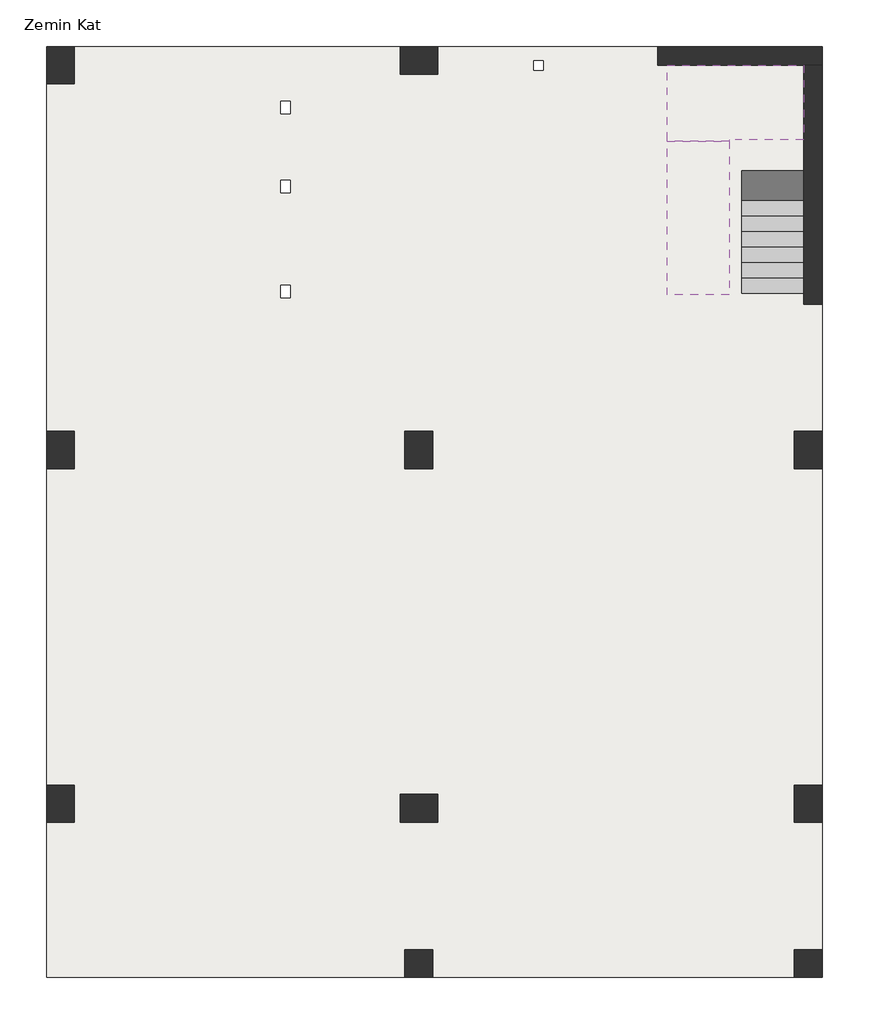
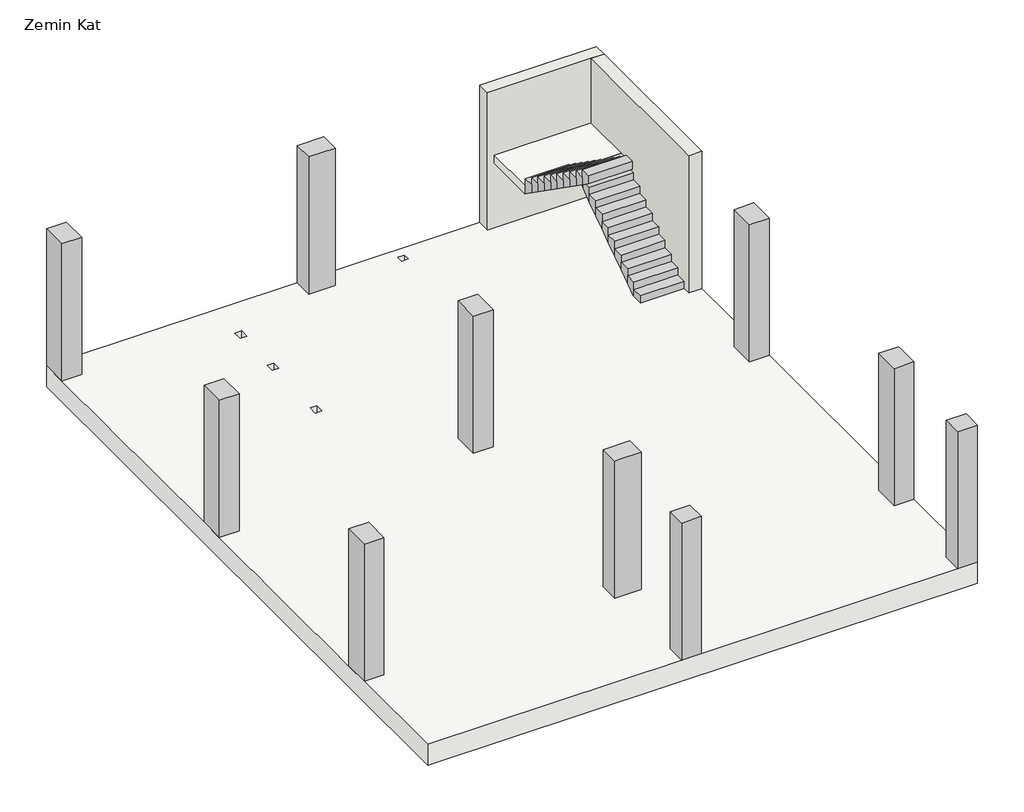
# One storey: 10 columns, 2 slabs, 2 stair flights, 2 walls.
"""IFC4 building model written with IfcOpenShell, lengths in millimetres."""

from ifc_helpers import new_model, si_unit, frame, origin, place, context, project, spatial, polyline, outline, extrude, faceted_brep, element, save

model = new_model("IFC4")

# Units and contexts
model_context = context("Model", 3, world=origin())
ifc_project = project(units=[si_unit("LENGTHUNIT", "METRE", prefix="MILLI")], contexts=[model_context])

# Site, building, storey
site = spatial("IfcSite", under=ifc_project)
building = spatial("IfcBuilding", under=site)
storey = spatial("IfcBuildingStorey", under=building, Name="Zemin Kat", Elevation=93780.0)

# Columns
placement = place(None, origin())
element("IfcColumn", 1, ObjectType="M_Concrete-Rectangular-Column : 450 x 450mm", at=placement, inside=storey, context=model_context, shape_type="SweptSolid", body=[
    extrude(outline(polyline([(-8954.0485128, -6221.7095574), (-9404.0485128, -6221.7095574), (-9404.0485128, -5771.7095574), (-8954.0485128, -5771.7095574), (-8954.0485128, -6221.7095574)])), frame((0.0, 0.0, 93780.0), z_axis=(0.0, 0.0, 1.0), x_axis=(1.0, 0.0, 0.0)), (0.0, 0.0, 1.0), 3300.0),
])
element("IfcColumn", 2, ObjectType="M_Concrete-Rectangular-Column : 450 x 450mm", at=placement, inside=storey, context=model_context, shape_type="SweptSolid", body=[
    extrude(outline(polyline([(-3129.0485128, -6221.7095574), (-3129.0485128, -5771.7095574), (-2679.0485128, -5771.7095574), (-2679.0485128, -6221.7095574), (-3129.0485128, -6221.7095574)])), frame((0.0, 0.0, 93780.0), z_axis=(0.0, 0.0, 1.0), x_axis=(1.0, 0.0, 0.0)), (0.0, 0.0, 1.0), 3300.0),
])
element("IfcColumn", 3, ObjectType="M_Concrete-Rectangular-Column : 450 x 600mm", at=placement, inside=storey, context=model_context, shape_type="SweptSolid", body=[
    extrude(outline(polyline([(-15179.0485128, -3721.7095574), (-15179.0485128, -3121.7095574), (-14729.0485128, -3121.7095574), (-14729.0485128, -3721.7095574), (-15179.0485128, -3721.7095574)])), frame((0.0, 0.0, 93780.0), z_axis=(0.0, 0.0, 1.0), x_axis=(1.0, 0.0, 0.0)), (0.0, 0.0, 1.0), 3300.0),
])
element("IfcColumn", 4, ObjectType="M_Concrete-Rectangular-Column : 450 x 600mm", at=placement, inside=storey, context=model_context, shape_type="SweptSolid", body=[
    extrude(outline(polyline([(-15179.0485128, 1978.2904426), (-15179.0485128, 2578.2904426), (-14729.0485128, 2578.2904426), (-14729.0485128, 1978.2904426), (-15179.0485128, 1978.2904426)])), frame((0.0, 0.0, 93780.0), z_axis=(0.0, 0.0, 1.0), x_axis=(1.0, 0.0, 0.0)), (0.0, 0.0, 1.0), 3300.0),
])
element("IfcColumn", 5, ObjectType="M_Concrete-Rectangular-Column : 450 x 600mm", at=placement, inside=storey, context=model_context, shape_type="SweptSolid", body=[
    extrude(outline(polyline([(-15179.0485128, 8178.2904426), (-15179.0485128, 8778.2904426), (-14729.0485128, 8778.2904426), (-14729.0485128, 8178.2904426), (-15179.0485128, 8178.2904426)])), frame((0.0, 0.0, 93780.0), z_axis=(0.0, 0.0, 1.0), x_axis=(1.0, 0.0, 0.0)), (0.0, 0.0, 1.0), 3300.0),
])
element("IfcColumn", 6, ObjectType="M_Concrete-Rectangular-Column : 450 x 600mm", at=placement, inside=storey, context=model_context, shape_type="Brep", body=[
    faceted_brep([(-8879.0485128, -3721.7095574, 93780.0), (-9479.0485128, -3721.7095574, 93780.0), (-9479.0485128, -3271.7095574, 93780.0), (-8879.0485128, -3271.7095574, 93780.0), (-8879.0485128, -3721.7095574, 97080.0), (-9404.0485128, -3721.7095574, 97080.0), (-9479.0485128, -3721.7095574, 97080.0), (-9479.0485128, -3271.7095574, 97080.0), (-8879.0485128, -3271.7095574, 97080.0)], [[[0, 1, 2, 3]], [[1, 0, 4, 5, 6]], [[2, 1, 6, 7]], [[3, 2, 7, 8]], [[0, 3, 8, 4]], [[6, 5, 4, 8, 7]]]),
])
element("IfcColumn", 7, ObjectType="M_Concrete-Rectangular-Column : 450 x 600mm", at=placement, inside=storey, context=model_context, shape_type="SweptSolid", body=[
    extrude(outline(polyline([(-9404.0485128, 1978.2904426), (-9404.0485128, 2578.2904426), (-8954.0485128, 2578.2904426), (-8954.0485128, 1978.2904426), (-9404.0485128, 1978.2904426)])), frame((0.0, 0.0, 93780.0), z_axis=(0.0, 0.0, 1.0), x_axis=(1.0, 0.0, 0.0)), (0.0, 0.0, 1.0), 3300.0),
])
element("IfcColumn", 8, ObjectType="M_Concrete-Rectangular-Column : 450 x 600mm", at=placement, inside=storey, context=model_context, shape_type="SweptSolid", body=[
    extrude(outline(polyline([(-8879.0485128, 8328.2904426), (-9479.0485128, 8328.2904426), (-9479.0485128, 8778.2904426), (-8879.0485128, 8778.2904426), (-8879.0485128, 8328.2904426)])), frame((0.0, 0.0, 93780.0), z_axis=(0.0, 0.0, 1.0), x_axis=(1.0, 0.0, 0.0)), (0.0, 0.0, 1.0), 3300.0),
])
element("IfcColumn", 9, ObjectType="M_Concrete-Rectangular-Column : 450 x 600mm", at=placement, inside=storey, context=model_context, shape_type="Brep", body=[
    faceted_brep([(-3129.0485128, -3721.7095574, 93780.0), (-3129.0485128, -3121.7095574, 93780.0), (-2679.0485128, -3121.7095574, 93780.0), (-2679.0485128, -3721.7095574, 93780.0), (-3129.0485128, -3721.7095574, 97080.0), (-3129.0485128, -3121.7095574, 97080.0), (-3129.0485128, -3121.7095574, 96680.0), (-2679.0485128, -3121.7095574, 97080.0), (-2679.0485128, -3121.7095574, 96680.0), (-2679.0485128, -3721.7095574, 97080.0)], [[[0, 1, 2, 3]], [[1, 0, 4, 5, 6]], [[2, 1, 6, 5, 7, 8]], [[3, 2, 8, 7, 9]], [[0, 3, 9, 4]], [[5, 4, 9, 7]]]),
])
element("IfcColumn", 10, ObjectType="M_Concrete-Rectangular-Column : 450 x 600mm", at=placement, inside=storey, context=model_context, shape_type="SweptSolid", body=[
    extrude(outline(polyline([(-3129.0485128, 1978.2904426), (-3129.0485128, 2578.2904426), (-2679.0485128, 2578.2904426), (-2679.0485128, 1978.2904426), (-3129.0485128, 1978.2904426)])), frame((0.0, 0.0, 93780.0), z_axis=(0.0, 0.0, 1.0), x_axis=(1.0, 0.0, 0.0)), (0.0, 0.0, 1.0), 3300.0),
])

# Slabs
element("IfcSlab", 11, ObjectType="200 mm Thickness", at=placement, inside=storey, context=model_context, shape_type="Brep", body=[
    faceted_brep([(-3979.0485128, 7278.2904426, 95530.0), (-2979.0485128, 7278.2904426, 95530.0), (-2979.0485128, 7279.1452058, 95530.0), (-2979.0485128, 8478.2904426, 95530.0), (-5179.0485128, 8478.2904426, 95530.0), (-5179.0485128, 7278.2904426, 95530.0), (-5179.0485128, 7277.4356794, 95530.0), (-5179.0485128, 7253.2904426, 95530.0), (-4179.0485128, 7253.2904426, 95530.0), (-4179.0485128, 7277.4356794, 95530.0), (-4179.0485128, 7278.2904426, 95530.0), (-5179.0485128, 8478.2904426, 95330.0), (-5179.0485128, 7278.2904426, 95330.0), (-5179.0485128, 7253.2904426, 95346.9016658), (-4179.0485128, 7253.2904426, 95346.9016658), (-5179.0485128, 7277.4356794, 95330.0), (-4179.0485128, 7278.2904426, 95330.0), (-3979.0485128, 7278.2904426, 95330.0), (-2979.0485128, 7278.2904426, 95329.4016658), (-2979.0485128, 7279.1452058, 95330.0), (-2979.0485128, 8478.2904426, 95330.0), (-3979.0485128, 7279.1452058, 95330.0), (-4179.0485128, 7277.4356794, 95330.0), (-3979.0485128, 7278.2904426, 95329.4016658)], [[[0, 1, 2, 3, 4, 5, 6, 7, 8, 9, 10]], [[5, 4, 11, 12]], [[8, 7, 13, 14]], [[5, 12, 15, 13, 7, 6]], [[0, 10, 16, 17]], [[1, 18, 19, 20, 3, 2]], [[19, 21, 17, 16, 22, 15, 12, 11, 20]], [[1, 0, 17, 23, 18]], [[4, 3, 20, 11]], [[8, 14, 22, 16, 10, 9]], [[21, 19, 18, 23]], [[17, 21, 23]], [[15, 22, 14, 13]]]),
])
element("IfcSlab", 12, ObjectType="Generic 500mm", at=placement, inside=storey, context=model_context, shape_type="Brep", body=[
    faceted_brep([(-2679.0485128, 8778.2904426, 93280.0), (-2679.0485128, -6221.7095574, 93280.0), (-15179.0485128, -6221.7095574, 93280.0), (-15179.0485128, 8778.2904426, 93280.0), (-11404.0485128, 6624.8694152, 93280.0), (-11404.0485128, 6424.8694152, 93280.0), (-11254.0485128, 6424.8694152, 93280.0), (-11254.0485128, 6624.8694152, 93280.0), (-11404.0485128, 4933.2654426, 93280.0), (-11404.0485128, 4733.2654426, 93280.0), (-11254.0485128, 4733.2654426, 93280.0), (-11254.0485128, 4933.2654426, 93280.0), (-11404.0485128, 7898.2904426, 93280.0), (-11404.0485128, 7698.2904426, 93280.0), (-11254.0485128, 7698.2904426, 93280.0), (-11254.0485128, 7898.2904426, 93280.0), (-7326.5485128, 8548.2904426, 93280.0), (-7326.5485128, 8398.2904426, 93280.0), (-7176.5485128, 8398.2904426, 93280.0), (-7176.5485128, 8548.2904426, 93280.0), (-2679.0485128, -6221.7095574, 93780.0), (-2679.0485128, -5771.7095574, 93780.0), (-2679.0485128, -3721.7095574, 93780.0), (-2679.0485128, -3121.7095574, 93780.0), (-2679.0485128, 1978.2904426, 93780.0), (-2679.0485128, 2578.2904426, 93780.0), (-2679.0485128, 8778.2904426, 93780.0), (-8879.0485128, 8778.2904426, 93780.0), (-9479.0485128, 8778.2904426, 93780.0), (-14729.0485128, 8778.2904426, 93780.0), (-15179.0485128, 8778.2904426, 93780.0), (-15179.0485128, 8178.2904426, 93780.0), (-15179.0485128, 2578.2904426, 93780.0), (-15179.0485128, 1978.2904426, 93780.0), (-15179.0485128, -3121.7095574, 93780.0), (-15179.0485128, -3721.7095574, 93780.0), (-15179.0485128, -6221.7095574, 93780.0), (-9404.0485128, -6221.7095574, 93780.0), (-8954.0485128, -6221.7095574, 93780.0), (-3129.0485128, -6221.7095574, 93780.0), (-11404.0485128, 6424.8694152, 93780.0), (-11404.0485128, 6624.8694152, 93780.0), (-11254.0485128, 6624.8694152, 93780.0), (-11254.0485128, 6424.8694152, 93780.0), (-11404.0485128, 4733.2654426, 93780.0), (-11404.0485128, 4933.2654426, 93780.0), (-11254.0485128, 4933.2654426, 93780.0), (-11254.0485128, 4733.2654426, 93780.0), (-11404.0485128, 7698.2904426, 93780.0), (-11404.0485128, 7898.2904426, 93780.0), (-11254.0485128, 7898.2904426, 93780.0), (-11254.0485128, 7698.2904426, 93780.0), (-7326.5485128, 8398.2904426, 93780.0), (-7326.5485128, 8548.2904426, 93780.0), (-7176.5485128, 8548.2904426, 93780.0), (-7176.5485128, 8398.2904426, 93780.0)], [[[0, 1, 2, 3], [4, 5, 6, 7], [8, 9, 10, 11], [12, 13, 14, 15], [16, 17, 18, 19]], [[20, 21, 22, 23, 24, 25, 26, 27, 28, 29, 30, 31, 32, 33, 34, 35, 36, 37, 38, 39], [40, 41, 42, 43], [44, 45, 46, 47], [48, 49, 50, 51], [52, 53, 54, 55]], [[1, 0, 26, 25, 24, 23, 22, 21, 20]], [[2, 1, 20, 39, 38, 37, 36]], [[3, 2, 36, 35, 34, 33, 32, 31, 30]], [[0, 3, 30, 29, 28, 27, 26]], [[4, 41, 40, 5]], [[5, 40, 43, 6]], [[6, 43, 42, 7]], [[41, 4, 7, 42]], [[8, 45, 44, 9]], [[9, 44, 47, 10]], [[10, 47, 46, 11]], [[45, 8, 11, 46]], [[12, 49, 48, 13]], [[13, 48, 51, 14]], [[14, 51, 50, 15]], [[49, 12, 15, 50]], [[16, 53, 52, 17]], [[17, 52, 55, 18]], [[18, 55, 54, 19]], [[53, 16, 19, 54]]]),
])

# Stair flights
element("IfcStairFlight", 13, ObjectType="25 mm Nosing", at=placement, inside=storey, context=model_context, shape_type="Brep", body=[
    faceted_brep([(-4179.0485128, 7003.2904426, 95705.0), (-4179.0485128, 7253.2904426, 95705.0), (-5179.0485128, 7253.2904426, 95705.0), (-5179.0485128, 7003.2904426, 95705.0), (-4179.0485128, 7003.2904426, 95521.9016658), (-4179.0485128, 7253.2904426, 95346.9016658), (-5179.0485128, 7253.2904426, 95346.9016658), (-5179.0485128, 7003.2904426, 95521.9016658), (-4179.0485128, 6753.2904426, 95880.0), (-4179.0485128, 7003.2904426, 95880.0), (-5179.0485128, 7003.2904426, 95880.0), (-5179.0485128, 6753.2904426, 95880.0), (-4179.0485128, 6753.2904426, 95696.9016658), (-5179.0485128, 6753.2904426, 95696.9016658), (-4179.0485128, 6503.2904426, 96055.0), (-4179.0485128, 6753.2904426, 96055.0), (-5179.0485128, 6753.2904426, 96055.0), (-5179.0485128, 6503.2904426, 96055.0), (-4179.0485128, 6503.2904426, 95871.9016658), (-5179.0485128, 6503.2904426, 95871.9016658), (-4179.0485128, 6253.2904426, 96230.0), (-4179.0485128, 6503.2904426, 96230.0), (-5179.0485128, 6503.2904426, 96230.0), (-5179.0485128, 6253.2904426, 96230.0), (-4179.0485128, 6253.2904426, 96046.9016658), (-5179.0485128, 6253.2904426, 96046.9016658), (-4179.0485128, 6003.2904426, 96405.0), (-4179.0485128, 6253.2904426, 96405.0), (-5179.0485128, 6253.2904426, 96405.0), (-5179.0485128, 6003.2904426, 96405.0), (-4179.0485128, 6003.2904426, 96221.9016658), (-5179.0485128, 6003.2904426, 96221.9016658), (-4179.0485128, 5753.2904426, 96580.0), (-4179.0485128, 6003.2904426, 96580.0), (-5179.0485128, 6003.2904426, 96580.0), (-5179.0485128, 5753.2904426, 96580.0), (-4179.0485128, 5753.2904426, 96396.9016658), (-5179.0485128, 5753.2904426, 96396.9016658), (-4179.0485128, 5503.2904426, 96755.0), (-4179.0485128, 5753.2904426, 96755.0), (-5179.0485128, 5753.2904426, 96755.0), (-5179.0485128, 5503.2904426, 96755.0), (-4179.0485128, 5503.2904426, 96571.9016658), (-5179.0485128, 5503.2904426, 96571.9016658), (-4179.0485128, 5253.2904426, 96930.0), (-4179.0485128, 5503.2904426, 96930.0), (-5179.0485128, 5503.2904426, 96930.0), (-5179.0485128, 5253.2904426, 96930.0), (-4179.0485128, 5253.2904426, 96746.9016658), (-5179.0485128, 5253.2904426, 96746.9016658), (-4179.0485128, 5003.2904426, 97105.0), (-4179.0485128, 5253.2904426, 97105.0), (-5179.0485128, 5253.2904426, 97105.0), (-5179.0485128, 5003.2904426, 97105.0), (-4179.0485128, 5003.2904426, 96921.9016658), (-5179.0485128, 5003.2904426, 96921.9016658), (-4179.0485128, 4778.2904426, 97280.0), (-4179.0485128, 5003.2904426, 97280.0), (-5179.0485128, 5003.2904426, 97280.0), (-5179.0485128, 4778.2904426, 97280.0), (-4179.0485128, 4778.2904426, 97079.4016658), (-5179.0485128, 4778.2904426, 97079.4016658)], [[[0, 1, 2, 3]], [[1, 0, 4, 5]], [[2, 1, 5, 6]], [[3, 2, 6, 7]], [[8, 9, 10, 11]], [[9, 8, 12, 4, 0]], [[10, 9, 0, 3]], [[11, 10, 3, 7, 13]], [[14, 15, 16, 17]], [[15, 14, 18, 12, 8]], [[16, 15, 8, 11]], [[17, 16, 11, 13, 19]], [[20, 21, 22, 23]], [[21, 20, 24, 18, 14]], [[22, 21, 14, 17]], [[23, 22, 17, 19, 25]], [[26, 27, 28, 29]], [[27, 26, 30, 24, 20]], [[28, 27, 20, 23]], [[29, 28, 23, 25, 31]], [[32, 33, 34, 35]], [[33, 32, 36, 30, 26]], [[34, 33, 26, 29]], [[35, 34, 29, 31, 37]], [[38, 39, 40, 41]], [[39, 38, 42, 36, 32]], [[40, 39, 32, 35]], [[41, 40, 35, 37, 43]], [[44, 45, 46, 47]], [[45, 44, 48, 42, 38]], [[46, 45, 38, 41]], [[47, 46, 41, 43, 49]], [[50, 51, 52, 53]], [[51, 50, 54, 48, 44]], [[52, 51, 44, 47]], [[53, 52, 47, 49, 55]], [[56, 57, 58, 59]], [[57, 56, 60, 54, 50]], [[58, 57, 50, 53]], [[59, 58, 53, 55, 61]], [[56, 59, 61, 60]], [[5, 4, 12, 18, 24, 30, 36, 42, 48, 54, 60, 61, 55, 49, 43, 37, 31, 25, 19, 13, 7, 6]]]),
])
element("IfcStairFlight", 14, ObjectType="25 mm Nosing", at=placement, inside=storey, context=model_context, shape_type="Brep", body=[
    faceted_brep([(-3979.0485128, 5053.2904426, 93955.0), (-3979.0485128, 4803.2904426, 93955.0), (-2979.0485128, 4803.2904426, 93955.0), (-2979.0485128, 5053.2904426, 93955.0), (-3979.0485128, 5053.2904426, 93780.0), (-3979.0485128, 4803.2904426, 93780.0), (-2979.0485128, 4803.2904426, 93780.0), (-2979.0485128, 5053.2904426, 93780.0), (-3979.0485128, 5303.2904426, 94130.0), (-3979.0485128, 5053.2904426, 94130.0), (-2979.0485128, 5053.2904426, 94130.0), (-2979.0485128, 5303.2904426, 94130.0), (-3979.0485128, 5303.2904426, 93946.9016658), (-3979.0485128, 5064.8594915, 93780.0), (-2979.0485128, 5064.8594915, 93780.0), (-2979.0485128, 5303.2904426, 93946.9016658), (-3979.0485128, 5553.2904426, 94305.0), (-3979.0485128, 5303.2904426, 94305.0), (-2979.0485128, 5303.2904426, 94305.0), (-2979.0485128, 5553.2904426, 94305.0), (-3979.0485128, 5553.2904426, 94121.9016658), (-2979.0485128, 5553.2904426, 94121.9016658), (-3979.0485128, 5803.2904426, 94480.0), (-3979.0485128, 5553.2904426, 94480.0), (-2979.0485128, 5553.2904426, 94480.0), (-2979.0485128, 5803.2904426, 94480.0), (-3979.0485128, 5803.2904426, 94296.9016658), (-2979.0485128, 5803.2904426, 94296.9016658), (-3979.0485128, 6053.2904426, 94655.0), (-3979.0485128, 5803.2904426, 94655.0), (-2979.0485128, 5803.2904426, 94655.0), (-2979.0485128, 6053.2904426, 94655.0), (-3979.0485128, 6053.2904426, 94471.9016658), (-2979.0485128, 6053.2904426, 94471.9016658), (-3979.0485128, 6303.2904426, 94830.0), (-3979.0485128, 6053.2904426, 94830.0), (-2979.0485128, 6053.2904426, 94830.0), (-2979.0485128, 6303.2904426, 94830.0), (-3979.0485128, 6303.2904426, 94646.9016658), (-2979.0485128, 6303.2904426, 94646.9016658), (-3979.0485128, 6553.2904426, 95005.0), (-3979.0485128, 6303.2904426, 95005.0), (-2979.0485128, 6303.2904426, 95005.0), (-2979.0485128, 6553.2904426, 95005.0), (-3979.0485128, 6553.2904426, 94821.9016658), (-2979.0485128, 6553.2904426, 94821.9016658), (-3979.0485128, 6803.2904426, 95180.0), (-3979.0485128, 6553.2904426, 95180.0), (-2979.0485128, 6553.2904426, 95180.0), (-2979.0485128, 6803.2904426, 95180.0), (-3979.0485128, 6803.2904426, 94996.9016658), (-2979.0485128, 6803.2904426, 94996.9016658), (-3979.0485128, 7053.2904426, 95355.0), (-3979.0485128, 6803.2904426, 95355.0), (-2979.0485128, 6803.2904426, 95355.0), (-2979.0485128, 7053.2904426, 95355.0), (-3979.0485128, 7053.2904426, 95171.9016658), (-2979.0485128, 7053.2904426, 95171.9016658), (-3979.0485128, 7278.2904426, 95530.0), (-3979.0485128, 7053.2904426, 95530.0), (-2979.0485128, 7053.2904426, 95530.0), (-2979.0485128, 7278.2904426, 95530.0), (-3979.0485128, 7278.2904426, 95330.0), (-3979.0485128, 7278.2904426, 95329.4016658), (-2979.0485128, 7278.2904426, 95329.4016658)], [[[0, 1, 2, 3]], [[1, 0, 4, 5]], [[2, 1, 5, 6]], [[3, 2, 6, 7]], [[8, 9, 10, 11]], [[4, 0, 9, 8, 12, 13]], [[0, 3, 10, 9]], [[3, 7, 14, 15, 11, 10]], [[16, 17, 18, 19]], [[17, 16, 20, 12, 8]], [[8, 11, 18, 17]], [[19, 18, 11, 15, 21]], [[22, 23, 24, 25]], [[23, 22, 26, 20, 16]], [[16, 19, 24, 23]], [[25, 24, 19, 21, 27]], [[28, 29, 30, 31]], [[29, 28, 32, 26, 22]], [[22, 25, 30, 29]], [[31, 30, 25, 27, 33]], [[34, 35, 36, 37]], [[35, 34, 38, 32, 28]], [[28, 31, 36, 35]], [[37, 36, 31, 33, 39]], [[40, 41, 42, 43]], [[41, 40, 44, 38, 34]], [[34, 37, 42, 41]], [[43, 42, 37, 39, 45]], [[46, 47, 48, 49]], [[47, 46, 50, 44, 40]], [[40, 43, 48, 47]], [[49, 48, 43, 45, 51]], [[52, 53, 54, 55]], [[53, 52, 56, 50, 46]], [[46, 49, 54, 53]], [[55, 54, 49, 51, 57]], [[58, 59, 60, 61]], [[59, 58, 62, 63, 56, 52]], [[52, 55, 60, 59]], [[61, 60, 55, 57, 64]], [[58, 61, 64, 63, 62]], [[5, 4, 13, 14, 7, 6]], [[14, 13, 12, 20, 26, 32, 38, 44, 50, 56, 63, 64, 57, 51, 45, 39, 33, 27, 21, 15]]]),
])

# Walls
element("IfcWall", 15, ObjectType="Generic - 300mm", at=placement, inside=storey, context=model_context, shape_type="Brep", body=[
    faceted_brep([(-2679.0485128, 8778.2904426, 93780.0), (-5329.0485128, 8778.2904426, 93780.0), (-5329.0485128, 8778.2904426, 96680.0), (-5329.0485128, 8778.2904426, 97080.0), (-2679.0485128, 8778.2904426, 97080.0), (-2679.0485128, 8478.2904426, 93780.0), (-2679.0485128, 8478.2904426, 97080.0), (-2979.0485128, 8478.2904426, 97080.0), (-5329.0485128, 8478.2904426, 97080.0), (-5329.0485128, 8478.2904426, 96680.0), (-5329.0485128, 8478.2904426, 93780.0), (-2979.0485128, 8478.2904426, 93780.0)], [[[0, 1, 2, 3, 4]], [[5, 6, 7, 8, 9, 10, 11]], [[1, 0, 5, 11, 10]], [[3, 2, 1, 10, 9, 8]], [[4, 3, 8, 7, 6]], [[0, 4, 6, 5]]]),
])
element("IfcWall", 16, ObjectType="Generic - 300mm", at=placement, inside=storey, context=model_context, shape_type="SweptSolid", body=[
    extrude(outline(polyline([(-2979.0485128, 4628.2904426), (-2979.0485128, 8478.2904426), (-2679.0485128, 8478.2904426), (-2679.0485128, 4628.2904426), (-2979.0485128, 4628.2904426)])), frame((0.0, 0.0, 93780.0), z_axis=(0.0, 0.0, 1.0), x_axis=(1.0, 0.0, 0.0)), (0.0, 0.0, 1.0), 3300.0),
])

save(model, "model.ifc")

# Revit data of these elements
# Project information
#   Project Issue Date = "Issue Date"
#   Project Status = "Project Status"
#   Client Name = "Owner"
#   Project Address = "Enter address here"
#   Project Name = "Project Name"
#   Project Number = "Project Number"
# Grids (mm)
#   "D": line (-18438.838, 8778.29) -> (-351.149, 8778.29)
#   "1": line (-15179.049, -7668.065) -> (-15179.049, 10376.164)
#   "2": line (-9179.049, -7668.065) -> (-9179.049, 10376.164)
#   "3": line (-2679.049, -7668.065) -> (-2679.049, 10376.164)
#   "A": line (-18438.838, -6221.71) -> (-351.149, -6221.71)
#   "B": line (-18438.838, -3721.71) -> (-351.149, -3721.71)
#   "C": line (-18438.838, 2278.29) -> (-351.149, 2278.29)
# Type "M_Concrete-Rectangular-Column : 450 x 450mm"
#   b = 45 cm
#   h = 45 cm
#   Structural Material [instance default] = Concrete, Cast-in-Place gray
# Type "M_Concrete-Rectangular-Column : 450 x 600mm"
#   b = 45 cm
#   h = 60 cm
#   Structural Material [instance default] = Concrete, Cast-in-Place gray
# Type "Generic 500mm"
#   Function = 0
#   Layers, outside or top first: 50 cm "Concrete, Cast-in-Place gray" (function 1)
# Type "Generic - 300mm"
#   Layers, outside or top first: 30 cm "Concrete, Cast-in-Place gray" (function 1)
# Elements 1, 2 (IfcColumn, "M_Concrete-Rectangular-Column : 450 x 450mm")
#   Structural Material = Concrete, Cast-in-Place gray
#   Phase Created = New Construction
#   Materials on its faces: "Concrete, Cast-in-Place gray"
# Elements 3, 4, 5, 6, 7, 8, 9, 10 (IfcColumn, "M_Concrete-Rectangular-Column : 450 x 600mm")
#   Structural Material = Concrete, Cast-in-Place gray
#   Phase Created = New Construction
#   Materials on its faces: "Concrete, Cast-in-Place gray"
# Element 11 (IfcSlab, "200 mm Thickness")
#   Phase Created = New Construction
#   Materials on its faces: "Concrete, Cast In Situ"
# Element 12 (IfcSlab, "Generic 500mm")
#   Height Offset From Level = 0 cm
#   built-in parameter 1001954 = 1
#   Phase Created = New Construction
#   Materials on its faces: "Concrete, Cast-in-Place gray"
# Elements 13, 14 (IfcStairFlight, "25 mm Nosing")
#   Phase Created = New Construction
#   Materials on its faces: "Concrete, Cast In Situ"
# Elements 15, 16 (IfcWall, "Generic - 300mm")
#   Comments = ""
#   Top Offset = -20 cm
#   Base Offset = 0 cm
#   wall height = 330 cm
#   Phase Created = New Construction
#   Base Constraint = Zemin Kat
#   Top Constraint = 1. Kat
#   Materials on its faces: "Concrete, Cast-in-Place gray"
# Materials
#   "Concrete, Cast-in-Place gray": class "Concrete", colour RGB 192 192 192, transparency 0, Description = "Cast-in-place concrete", Cost = 0
#   "Concrete, Cast In Situ": class "Concrete", colour RGB 192 192 192, transparency 0, Description = "physical material", Cost = 0
